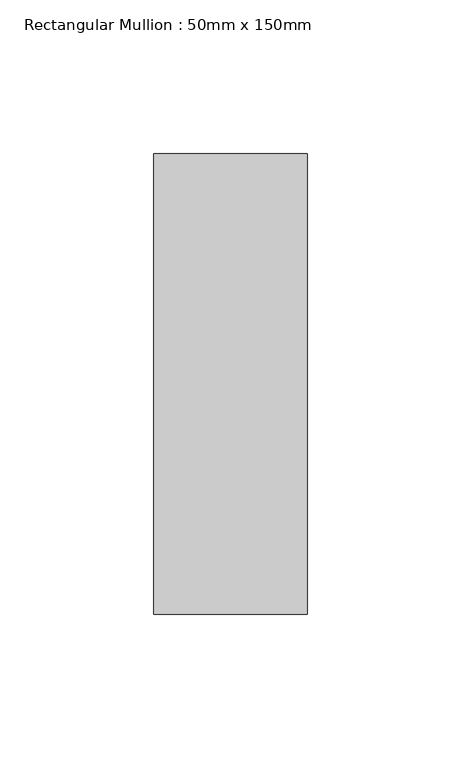
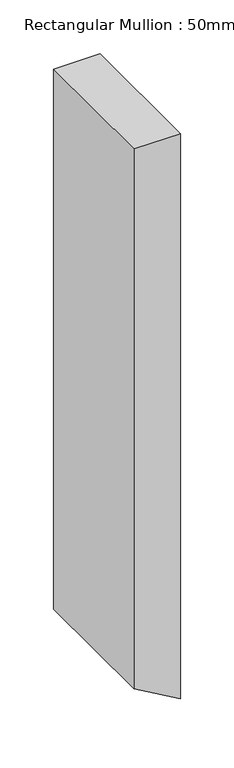
"""IFC4 building model written with IfcOpenShell, lengths in millimetres: member geometry, Rectangular Mullion : 50mm x 150mm."""

from ifc_helpers import new_model, si_unit, frame, origin, place, context, project, spatial, polyline, outline, extrude, source, transform, mapped, element, save


def rectangular_mullion_50mm_x_150mm_b704ab83(model_context):
    return source(origin(), model_context, "Body", "SweptSolid", [
        extrude(outline(polyline([(0.0, 0.0), (0.0, -50.0), (-614.5081595, -50.0), (-643.375673, 0.0), (0.0, 0.0)])), frame((0.0, -75.0, 0.0), z_axis=(0.0, 1.0, 0.0), x_axis=(0.0, 0.0, 1.0)), (0.0, 0.0, 1.0), 150.0),
    ])


if __name__ == "__main__":
    model = new_model("IFC4")
    model_context = context("Model", 3, world=origin())
    ifc_project = project(units=[si_unit("LENGTHUNIT", "METRE", prefix="MILLI")], contexts=[model_context])
    site = spatial("IfcSite", under=ifc_project)
    building = spatial("IfcBuilding", under=site)
    placement = place(None, origin())
    rectangular_mullion_50mm_x_150mm_shape = rectangular_mullion_50mm_x_150mm_b704ab83(model_context)
    element("IfcMember", 1, ObjectType="Rectangular Mullion : 50mm x 150mm", at=placement, inside=building, context=model_context, shape_type="MappedRepresentation", body=[
        mapped(rectangular_mullion_50mm_x_150mm_shape, transform((0.0, 0.0, 0.0), x_axis=(1.0, 0.0, 0.0), y_axis=(0.0, 1.0, 0.0), z_axis=(0.0, 0.0, 1.0))),
    ])
    save(model, "model.ifc")

# Revit data of these elements
# Type "Rectangular Mullion : 50mm x 150mm"
#   built-in parameter 1007304 = 0.492126 (stored number, unit not read)
#   built-in parameter 1007301 = 0.082021 (stored number, unit not read)
#   built-in parameter 1007300 = 0.082021 (stored number, unit not read)
# Element 1 (IfcMember, "Rectangular Mullion : 50mm x 150mm")
#   Materials on its faces: "Aluminum"
# Materials
#   "Aluminum": class "Metal", colour RGB 247 247 247, transparency 0, Description = "Aluminum 6061", Cost = 0
